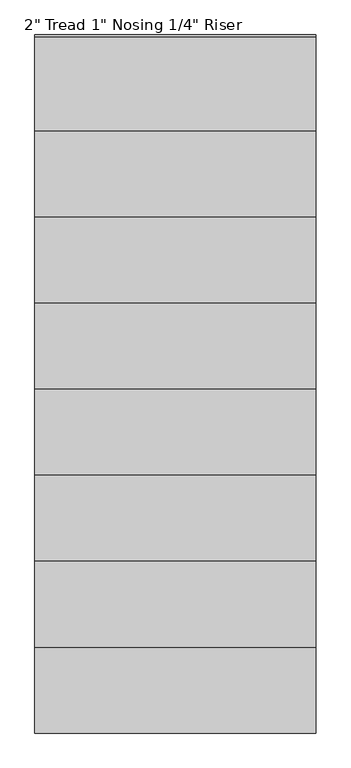
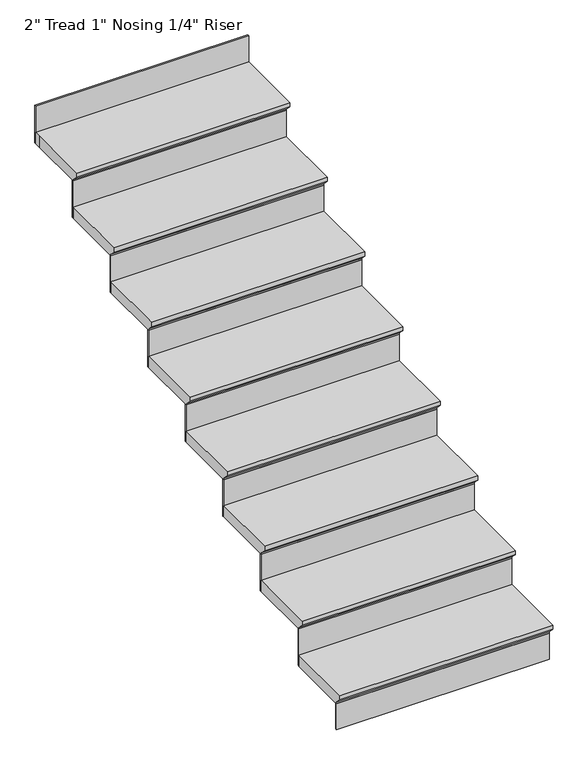
"""IFC4 building model written with IfcOpenShell, lengths in millimetres: stair flight geometry."""

from ifc_helpers import new_model, si_unit, origin, place, context, project, spatial, faceted_brep, source, transform, mapped, element, save


def stair_flight_15e98d73(model_context):
    return source(origin(), model_context, "Body", "Brep", [
        faceted_brep([(14913.1123343, 14886.0483822, 169.3333333), (15827.5123343, 14886.0483822, 169.3333333), (15827.5123343, 15190.8483822, 169.3333333), (14913.1123343, 15190.8483822, 169.3333333), (14913.1123343, 14911.4483822, 118.5333333), (14913.1123343, 15190.8483822, 118.5333333), (15827.5123343, 15190.8483822, 118.5333333), (15827.5123343, 14911.4483822, 118.5333333), (14913.1123343, 14911.4483822, 124.8833333), (14913.1123343, 14886.0483822, 150.2833333), (15827.5123343, 14911.4483822, 124.8833333), (15827.5123343, 14886.0483822, 150.2833333)], [[[0, 1, 2, 3]], [[4, 5, 6, 7]], [[0, 3, 5, 4, 8, 9]], [[4, 7, 10, 8]], [[2, 1, 11, 10, 7, 6]], [[3, 2, 6, 5]], [[11, 1, 0, 9]], [[10, 11, 9, 8]]]),
        faceted_brep([(15827.5123343, 14911.4483822, 118.5333333), (15827.5123343, 14911.4483822, 0.0), (15827.5123343, 14917.7983822, 0.0), (15827.5123343, 14917.7983822, 118.5333333), (14913.1123343, 14911.4483822, 118.5333333), (14913.1123343, 14917.7983822, 118.5333333), (14913.1123343, 14917.7983822, 0.0), (14913.1123343, 14911.4483822, 0.0)], [[[0, 1, 2, 3]], [[4, 5, 6, 7]], [[1, 0, 4, 7]], [[2, 1, 7, 6]], [[3, 2, 6, 5]], [[0, 3, 5, 4]]]),
        faceted_brep([(14913.1123343, 15165.4483822, 338.6666667), (15827.5123343, 15165.4483822, 338.6666667), (15827.5123343, 15470.2483822, 338.6666667), (14913.1123343, 15470.2483822, 338.6666667), (14913.1123343, 15190.8483822, 287.8666667), (14913.1123343, 15470.2483822, 287.8666667), (15827.5123343, 15470.2483822, 287.8666667), (15827.5123343, 15190.8483822, 287.8666667), (14913.1123343, 15190.8483822, 294.2166667), (14913.1123343, 15165.4483822, 319.6166667), (15827.5123343, 15190.8483822, 294.2166667), (15827.5123343, 15165.4483822, 319.6166667)], [[[0, 1, 2, 3]], [[4, 5, 6, 7]], [[0, 3, 5, 4, 8, 9]], [[4, 7, 10, 8]], [[2, 1, 11, 10, 7, 6]], [[3, 2, 6, 5]], [[11, 1, 0, 9]], [[10, 11, 9, 8]]]),
        faceted_brep([(15827.5123343, 15190.8483822, 287.8666667), (15827.5123343, 15190.8483822, 118.5333333), (15827.5123343, 15197.1983822, 118.5333333), (15827.5123343, 15197.1983822, 287.8666667), (14913.1123343, 15190.8483822, 287.8666667), (14913.1123343, 15197.1983822, 287.8666667), (14913.1123343, 15197.1983822, 118.5333333), (14913.1123343, 15190.8483822, 118.5333333)], [[[0, 1, 2, 3]], [[4, 5, 6, 7]], [[1, 0, 4, 7]], [[2, 1, 7, 6]], [[3, 2, 6, 5]], [[0, 3, 5, 4]]]),
        faceted_brep([(14913.1123343, 15444.8483822, 508.0), (15827.5123343, 15444.8483822, 508.0), (15827.5123343, 15749.6483822, 508.0), (14913.1123343, 15749.6483822, 508.0), (14913.1123343, 15470.2483822, 457.2), (14913.1123343, 15749.6483822, 457.2), (15827.5123343, 15749.6483822, 457.2), (15827.5123343, 15470.2483822, 457.2), (14913.1123343, 15470.2483822, 463.55), (14913.1123343, 15444.8483822, 488.95), (15827.5123343, 15470.2483822, 463.55), (15827.5123343, 15444.8483822, 488.95)], [[[0, 1, 2, 3]], [[4, 5, 6, 7]], [[0, 3, 5, 4, 8, 9]], [[4, 7, 10, 8]], [[2, 1, 11, 10, 7, 6]], [[3, 2, 6, 5]], [[11, 1, 0, 9]], [[10, 11, 9, 8]]]),
        faceted_brep([(15827.5123343, 15470.2483822, 457.2), (15827.5123343, 15470.2483822, 287.8666667), (15827.5123343, 15476.5983822, 287.8666667), (15827.5123343, 15476.5983822, 457.2), (14913.1123343, 15470.2483822, 457.2), (14913.1123343, 15476.5983822, 457.2), (14913.1123343, 15476.5983822, 287.8666667), (14913.1123343, 15470.2483822, 287.8666667)], [[[0, 1, 2, 3]], [[4, 5, 6, 7]], [[1, 0, 4, 7]], [[2, 1, 7, 6]], [[3, 2, 6, 5]], [[0, 3, 5, 4]]]),
        faceted_brep([(14913.1123343, 15724.2483822, 677.3333333), (15827.5123343, 15724.2483822, 677.3333333), (15827.5123343, 16029.0483822, 677.3333333), (14913.1123343, 16029.0483822, 677.3333333), (14913.1123343, 15749.6483822, 626.5333333), (14913.1123343, 16029.0483822, 626.5333333), (15827.5123343, 16029.0483822, 626.5333333), (15827.5123343, 15749.6483822, 626.5333333), (14913.1123343, 15749.6483822, 632.8833333), (14913.1123343, 15724.2483822, 658.2833333), (15827.5123343, 15749.6483822, 632.8833333), (15827.5123343, 15724.2483822, 658.2833333)], [[[0, 1, 2, 3]], [[4, 5, 6, 7]], [[0, 3, 5, 4, 8, 9]], [[4, 7, 10, 8]], [[2, 1, 11, 10, 7, 6]], [[3, 2, 6, 5]], [[11, 1, 0, 9]], [[10, 11, 9, 8]]]),
        faceted_brep([(15827.5123343, 15749.6483822, 626.5333333), (15827.5123343, 15749.6483822, 457.2), (15827.5123343, 15755.9983822, 457.2), (15827.5123343, 15755.9983822, 626.5333333), (14913.1123343, 15749.6483822, 626.5333333), (14913.1123343, 15755.9983822, 626.5333333), (14913.1123343, 15755.9983822, 457.2), (14913.1123343, 15749.6483822, 457.2)], [[[0, 1, 2, 3]], [[4, 5, 6, 7]], [[1, 0, 4, 7]], [[2, 1, 7, 6]], [[3, 2, 6, 5]], [[0, 3, 5, 4]]]),
        faceted_brep([(14913.1123343, 16003.6483822, 846.6666667), (15827.5123343, 16003.6483822, 846.6666667), (15827.5123343, 16308.4483822, 846.6666667), (14913.1123343, 16308.4483822, 846.6666667), (14913.1123343, 16029.0483822, 795.8666667), (14913.1123343, 16308.4483822, 795.8666667), (15827.5123343, 16308.4483822, 795.8666667), (15827.5123343, 16029.0483822, 795.8666667), (14913.1123343, 16029.0483822, 802.2166667), (14913.1123343, 16003.6483822, 827.6166667), (15827.5123343, 16029.0483822, 802.2166667), (15827.5123343, 16003.6483822, 827.6166667)], [[[0, 1, 2, 3]], [[4, 5, 6, 7]], [[0, 3, 5, 4, 8, 9]], [[4, 7, 10, 8]], [[2, 1, 11, 10, 7, 6]], [[3, 2, 6, 5]], [[11, 1, 0, 9]], [[10, 11, 9, 8]]]),
        faceted_brep([(15827.5123343, 16029.0483822, 795.8666667), (15827.5123343, 16029.0483822, 626.5333333), (15827.5123343, 16035.3983822, 626.5333333), (15827.5123343, 16035.3983822, 795.8666667), (14913.1123343, 16029.0483822, 795.8666667), (14913.1123343, 16035.3983822, 795.8666667), (14913.1123343, 16035.3983822, 626.5333333), (14913.1123343, 16029.0483822, 626.5333333)], [[[0, 1, 2, 3]], [[4, 5, 6, 7]], [[1, 0, 4, 7]], [[2, 1, 7, 6]], [[3, 2, 6, 5]], [[0, 3, 5, 4]]]),
        faceted_brep([(14913.1123343, 16283.0483822, 1016.0), (15827.5123343, 16283.0483822, 1016.0), (15827.5123343, 16587.8483822, 1016.0), (14913.1123343, 16587.8483822, 1016.0), (14913.1123343, 16308.4483822, 965.2), (14913.1123343, 16587.8483822, 965.2), (15827.5123343, 16587.8483822, 965.2), (15827.5123343, 16308.4483822, 965.2), (14913.1123343, 16308.4483822, 971.55), (14913.1123343, 16283.0483822, 996.95), (15827.5123343, 16308.4483822, 971.55), (15827.5123343, 16283.0483822, 996.95)], [[[0, 1, 2, 3]], [[4, 5, 6, 7]], [[0, 3, 5, 4, 8, 9]], [[4, 7, 10, 8]], [[2, 1, 11, 10, 7, 6]], [[3, 2, 6, 5]], [[11, 1, 0, 9]], [[10, 11, 9, 8]]]),
        faceted_brep([(15827.5123343, 16308.4483822, 965.2), (15827.5123343, 16308.4483822, 795.8666667), (15827.5123343, 16314.7983822, 795.8666667), (15827.5123343, 16314.7983822, 965.2), (14913.1123343, 16308.4483822, 965.2), (14913.1123343, 16314.7983822, 965.2), (14913.1123343, 16314.7983822, 795.8666667), (14913.1123343, 16308.4483822, 795.8666667)], [[[0, 1, 2, 3]], [[4, 5, 6, 7]], [[1, 0, 4, 7]], [[2, 1, 7, 6]], [[3, 2, 6, 5]], [[0, 3, 5, 4]]]),
        faceted_brep([(14913.1123343, 16562.4483822, 1185.3333333), (15827.5123343, 16562.4483822, 1185.3333333), (15827.5123343, 16867.2483822, 1185.3333333), (14913.1123343, 16867.2483822, 1185.3333333), (14913.1123343, 16587.8483822, 1134.5333333), (14913.1123343, 16867.2483822, 1134.5333333), (15827.5123343, 16867.2483822, 1134.5333333), (15827.5123343, 16587.8483822, 1134.5333333), (14913.1123343, 16587.8483822, 1140.8833333), (14913.1123343, 16562.4483822, 1166.2833333), (15827.5123343, 16587.8483822, 1140.8833333), (15827.5123343, 16562.4483822, 1166.2833333)], [[[0, 1, 2, 3]], [[4, 5, 6, 7]], [[0, 3, 5, 4, 8, 9]], [[4, 7, 10, 8]], [[2, 1, 11, 10, 7, 6]], [[3, 2, 6, 5]], [[11, 1, 0, 9]], [[10, 11, 9, 8]]]),
        faceted_brep([(15827.5123343, 16587.8483822, 1134.5333333), (15827.5123343, 16587.8483822, 965.2), (15827.5123343, 16594.1983822, 965.2), (15827.5123343, 16594.1983822, 1134.5333333), (14913.1123343, 16587.8483822, 1134.5333333), (14913.1123343, 16594.1983822, 1134.5333333), (14913.1123343, 16594.1983822, 965.2), (14913.1123343, 16587.8483822, 965.2)], [[[0, 1, 2, 3]], [[4, 5, 6, 7]], [[1, 0, 4, 7]], [[2, 1, 7, 6]], [[3, 2, 6, 5]], [[0, 3, 5, 4]]]),
        faceted_brep([(14913.1123343, 17146.6483822, 1354.6666667), (14913.1123343, 17121.2483822, 1354.6666667), (14913.1123343, 16841.8483822, 1354.6666667), (15827.5123343, 16841.8483822, 1354.6666667), (15827.5123343, 17146.6483822, 1354.6666667), (14913.1123343, 17121.2483822, 1303.8666667), (14913.1123343, 17146.6483822, 1303.8666667), (15827.5123343, 17146.6483822, 1303.8666667), (15827.5123343, 16867.2483822, 1303.8666667), (14913.1123343, 16867.2483822, 1303.8666667), (15827.5123343, 16867.2483822, 1310.2166667), (14913.1123343, 16867.2483822, 1310.2166667), (15827.5123343, 16841.8483822, 1335.6166667), (14913.1123343, 16841.8483822, 1335.6166667)], [[[0, 1, 2, 3, 4]], [[5, 6, 7, 8, 9]], [[1, 0, 6, 5]], [[9, 8, 10, 11]], [[4, 3, 12, 10, 8, 7]], [[0, 4, 7, 6]], [[12, 3, 2, 13]], [[10, 12, 13, 11]], [[2, 1, 5, 9, 11, 13]]]),
        faceted_brep([(15827.5123343, 16867.2483822, 1303.8666667), (15827.5123343, 16867.2483822, 1134.5333333), (15827.5123343, 16873.5983822, 1134.5333333), (15827.5123343, 16873.5983822, 1303.8666667), (14913.1123343, 16867.2483822, 1303.8666667), (14913.1123343, 16873.5983822, 1303.8666667), (14913.1123343, 16873.5983822, 1134.5333333), (14913.1123343, 16867.2483822, 1134.5333333)], [[[0, 1, 2, 3]], [[4, 5, 6, 7]], [[1, 0, 4, 7]], [[2, 1, 7, 6]], [[3, 2, 6, 5]], [[0, 3, 5, 4]]]),
        faceted_brep([(15827.5123343, 17146.6483822, 1473.2), (15827.5123343, 17146.6483822, 1303.8666667), (15827.5123343, 17152.9983822, 1303.8666667), (15827.5123343, 17152.9983822, 1473.2), (14913.1123343, 17146.6483822, 1473.2), (14913.1123343, 17152.9983822, 1473.2), (14913.1123343, 17152.9983822, 1303.8666667), (14913.1123343, 17146.6483822, 1303.8666667)], [[[0, 1, 2, 3]], [[4, 5, 6, 7]], [[1, 0, 4, 7]], [[2, 1, 7, 6]], [[3, 2, 6, 5]], [[0, 3, 5, 4]]]),
    ])


if __name__ == "__main__":
    model = new_model("IFC4")
    model_context = context("Model", 3, world=origin())
    ifc_project = project(units=[si_unit("LENGTHUNIT", "METRE", prefix="MILLI")], contexts=[model_context])
    site = spatial("IfcSite", under=ifc_project)
    building = spatial("IfcBuilding", under=site)
    placement = place(None, origin())
    stair_flight_shape = stair_flight_15e98d73(model_context)
    element("IfcStairFlight", 1, ObjectType="2\" Tread 1\" Nosing 1/4\" Riser", at=placement, inside=building, context=model_context, shape_type="MappedRepresentation", body=[
        mapped(stair_flight_shape, transform((0.0, 0.0, 0.0), x_axis=(1.0, 0.0, 0.0), y_axis=(0.0, 1.0, 0.0), z_axis=(0.0, 0.0, 1.0))),
    ])
    save(model, "model.ifc")

# Revit data of these elements
# Element 1 (IfcStairFlight, "2\" Tread 1\" Nosing 1/4\" Riser")
#   Materials on its faces: "Oak Flooring"
# Materials
#   "Oak Flooring": class "Wood", colour RGB 216 169 114, transparency 0, Description = "Quercus Rubra", Cost = 0
